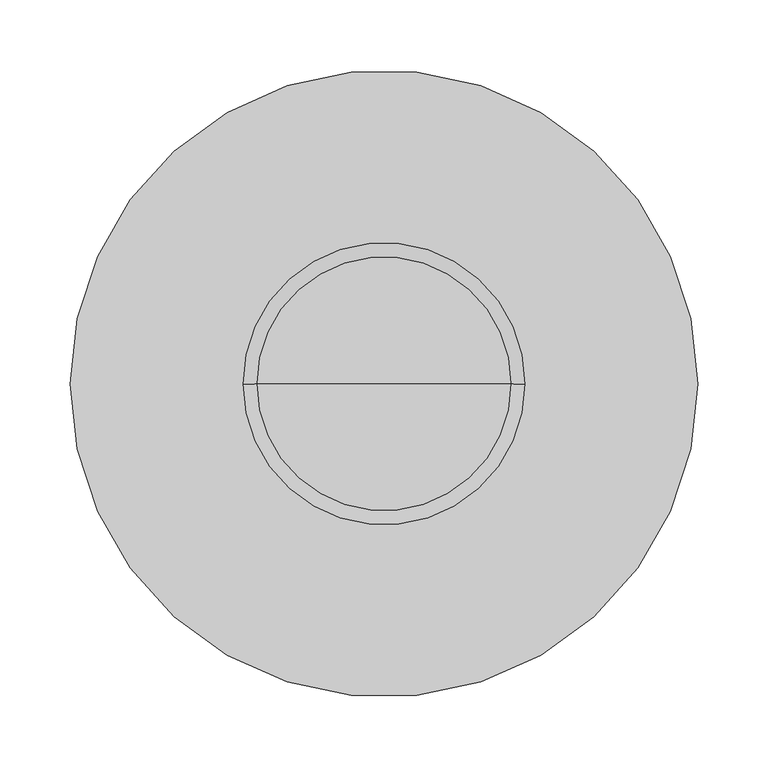
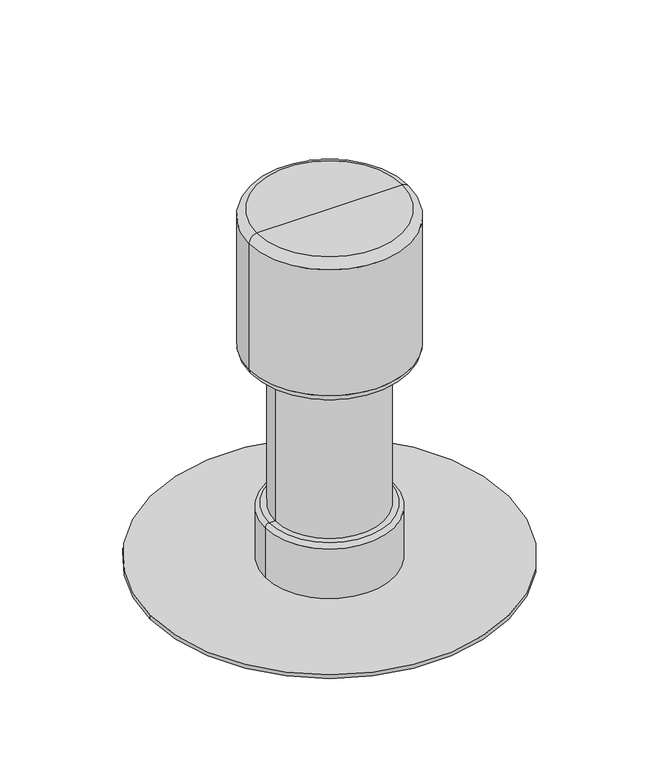
"""IFC4 building model written with IfcOpenShell, lengths in millimetres: proxy geometry, TN_Аэратор кровельный  ТехноНИКОЛЬ : Аэратор кровельный ТехноНИКОЛЬ 160х460мм."""

from ifc_helpers import new_model, si_unit, point, frame, origin, origin_with_axes, origin_2d, place, context, project, spatial, circle_curve, ellipse_curve, trimmed, segment, composite_curve, outline, extrude, source, transform, mapped, element, save
from ifc_brep_helpers import plane_surface, cylinder_surface, revolved_surface, advanced_brep


def specialty_equipment_49e8ba72(model_context):
    return source(origin(), model_context, "Body", "SolidModel", [
        advanced_brep(
        [(0.0, 0.0, 5.0), (-80.0, 0.0, 5.0), (80.0, 0.0, 5.0), (67.5, 0.0, 275.0), (-67.5, 0.0, 275.0), (0.0, 0.0, 275.0), (67.5, 0.0, 75.0), (-67.5, 0.0, 75.0), (75.0, 0.0, 75.0), (-75.0, 0.0, 75.0), (80.0, 0.0, 70.0), (-80.0, 0.0, 70.0)],
        [
            (0, 1),
            (1, 2, circle_curve(frame((0.0, 0.0, 5.0), z_axis=(0.0, 0.0, -1.0), x_axis=(-1.0, 0.0, 0.0)), 80.0)),
            (2, 0),
            (2, 1, circle_curve(frame((0.0, 0.0, 5.0), z_axis=(0.0, 0.0, -1.0), x_axis=(-1.0, 0.0, 0.0)), 80.0)),
            (3, 4, circle_curve(frame((0.0, 0.0, 275.0), z_axis=(0.0, 0.0, 1.0), x_axis=(-1.0, 0.0, 0.0)), 67.5)),
            (4, 5),
            (5, 3),
            (4, 3, circle_curve(frame((0.0, 0.0, 275.0), z_axis=(0.0, 0.0, 1.0), x_axis=(-1.0, 0.0, 0.0)), 67.5)),
            (6, 7, circle_curve(frame((0.0, 0.0, 75.0), z_axis=(0.0, 0.0, 1.0), x_axis=(-1.0, 0.0, 0.0)), 67.5)),
            (7, 4),
            (3, 6),
            (7, 6, circle_curve(frame((0.0, 0.0, 75.0), z_axis=(0.0, 0.0, 1.0), x_axis=(-1.0, 0.0, 0.0)), 67.5)),
            (8, 9, circle_curve(frame((0.0, 0.0, 75.0), z_axis=(0.0, 0.0, 1.0), x_axis=(-1.0, 0.0, 0.0)), 75.0)),
            (9, 7),
            (6, 8),
            (9, 8, circle_curve(frame((0.0, 0.0, 75.0), z_axis=(0.0, 0.0, 1.0), x_axis=(-1.0, 0.0, 0.0)), 75.0)),
            (10, 11, circle_curve(frame((0.0, 0.0, 70.0), z_axis=(0.0, 0.0, 1.0), x_axis=(-1.0, 0.0, 0.0)), 80.0)),
            (11, 9, circle_curve(frame((-75.0, 0.0, 70.0), z_axis=(0.0, 1.0, 0.0), x_axis=(1.0, 0.0, 0.0)), 5.0)),
            (8, 10, circle_curve(frame((75.0, 0.0, 70.0), z_axis=(0.0, 1.0, 0.0), x_axis=(-1.0, 0.0, 0.0)), 5.0)),
            (11, 10, circle_curve(frame((0.0, 0.0, 70.0), z_axis=(0.0, 0.0, 1.0), x_axis=(-1.0, 0.0, 0.0)), 80.0)),
            (1, 11),
            (10, 2),
        ],
        [
            plane_surface(frame((0.0, 0.0, 5.0), z_axis=(0.0, 0.0, -1.0), x_axis=(-1.0, 0.0, 0.0))),
            plane_surface(frame((0.0, 0.0, 275.0), z_axis=(0.0, 0.0, 1.0), x_axis=(-1.0, 0.0, 0.0))),
            cylinder_surface(frame((0.0, 0.0, 0.0), z_axis=(0.0, 0.0, -1.0), x_axis=(-1.0, 0.0, 0.0)), 67.5),
            plane_surface(frame((0.0, 0.0, 75.0), z_axis=(0.0, 0.0, 1.0), x_axis=(-1.0, 0.0, 0.0))),
            revolved_surface(trimmed(ellipse_curve(frame((-75.0, 0.0, 70.0), z_axis=(0.0, -1.0, 0.0), x_axis=(1.0, 0.0, 0.0)), 5.0, 5.0), [point((-75.0, 0.0, 75.0))], [point((-80.0, 0.0, 70.0))], True, "CARTESIAN"), (0.0, 0.0, 0.0), (0.0, 0.0, -1.0)),
            cylinder_surface(frame((0.0, 0.0, 0.0), z_axis=(0.0, 0.0, -1.0), x_axis=(-1.0, 0.0, 0.0)), 80.0),
        ],
        [
            (0, [[1, 2, 3]]),
            (0, [[-3, 4, -1]]),
            (1, [[5, 6, 7]]),
            (1, [[8, -7, -6]]),
            (2, [[9, 10, -5, 11]]),
            (2, [[12, -11, -8, -10]]),
            (3, [[13, 14, -9, 15]]),
            (3, [[16, -15, -12, -14]]),
            (4, [[17, 18, -13, 19]]),
            (4, [[20, -19, -16, -18]]),
            (5, [[-2, 21, -17, 22]]),
            (5, [[-4, -22, -20, -21]]),
        ],
    ),
        extrude(outline(composite_curve([segment(trimmed(circle_curve(origin_2d(), 222.5), [point((-222.5, 0.0))], [point((222.5, 0.0))], False, "CARTESIAN"), True, "CONTINUOUS"), segment(trimmed(circle_curve(origin_2d(), 222.5), [point((222.5, 0.0))], [point((-222.5, 0.0))], False, "CARTESIAN"), True, "CONTINUOUS")], self_intersect=False)), origin_with_axes(), (0.0, 0.0, 1.0), 5.0),
        advanced_brep(
        [(90.0, 0.0, 460.0), (-90.0, 0.0, 460.0), (0.0, 0.0, 460.0), (100.0, 0.0, 450.0), (-100.0, 0.0, 450.0), (100.0, 0.0, 285.0), (-100.0, 0.0, 285.0), (90.0, 0.0, 275.0), (-90.0, 0.0, 275.0), (0.0, 0.0, 275.0)],
        [
            (0, 1, circle_curve(frame((0.0, 0.0, 460.0), z_axis=(0.0, 0.0, 1.0), x_axis=(-1.0, 0.0, 0.0)), 90.0)),
            (1, 2),
            (2, 0),
            (1, 0, circle_curve(frame((0.0, 0.0, 460.0), z_axis=(0.0, 0.0, 1.0), x_axis=(-1.0, 0.0, 0.0)), 90.0)),
            (3, 4, circle_curve(frame((0.0, 0.0, 450.0), z_axis=(0.0, 0.0, 1.0), x_axis=(-1.0, 0.0, 0.0)), 100.0)),
            (4, 1, circle_curve(frame((-90.0, 0.0, 450.0), z_axis=(0.0, 1.0, 0.0), x_axis=(1.0, 0.0, 0.0)), 10.0)),
            (0, 3, circle_curve(frame((90.0, 0.0, 450.0), z_axis=(0.0, 1.0, 0.0), x_axis=(-1.0, 0.0, 0.0)), 10.0)),
            (4, 3, circle_curve(frame((0.0, 0.0, 450.0), z_axis=(0.0, 0.0, 1.0), x_axis=(-1.0, 0.0, 0.0)), 100.0)),
            (5, 6, circle_curve(frame((0.0, 0.0, 285.0), z_axis=(0.0, 0.0, 1.0), x_axis=(-1.0, 0.0, 0.0)), 100.0)),
            (6, 4),
            (3, 5),
            (6, 5, circle_curve(frame((0.0, 0.0, 285.0), z_axis=(0.0, 0.0, 1.0), x_axis=(-1.0, 0.0, 0.0)), 100.0)),
            (7, 8, circle_curve(frame((0.0, 0.0, 275.0), z_axis=(0.0, 0.0, 1.0), x_axis=(-1.0, 0.0, 0.0)), 90.0)),
            (8, 6, circle_curve(frame((-90.0, 0.0, 285.0), z_axis=(0.0, 1.0, 0.0), x_axis=(1.0, 0.0, 0.0)), 10.0)),
            (5, 7, circle_curve(frame((90.0, 0.0, 285.0), z_axis=(0.0, 1.0, 0.0), x_axis=(-1.0, 0.0, 0.0)), 10.0)),
            (8, 7, circle_curve(frame((0.0, 0.0, 275.0), z_axis=(0.0, 0.0, 1.0), x_axis=(-1.0, 0.0, 0.0)), 90.0)),
            (9, 8),
            (7, 9),
        ],
        [
            plane_surface(frame((0.0, 0.0, 460.0), z_axis=(0.0, 0.0, 1.0), x_axis=(-1.0, 0.0, 0.0))),
            revolved_surface(trimmed(ellipse_curve(frame((-90.0, 0.0, 450.0), z_axis=(0.0, -1.0, 0.0), x_axis=(1.0, 0.0, 0.0)), 10.0, 10.0), [point((-90.0, 0.0, 460.0))], [point((-100.0, 0.0, 450.0))], True, "CARTESIAN"), (0.0, 0.0, 460.0), (0.0, 0.0, -1.0)),
            cylinder_surface(frame((0.0, 0.0, 460.0), z_axis=(0.0, 0.0, -1.0), x_axis=(-1.0, 0.0, 0.0)), 100.0),
            revolved_surface(trimmed(ellipse_curve(frame((-90.0, 0.0, 285.0), z_axis=(0.0, -1.0, 0.0), x_axis=(1.0, 0.0, 0.0)), 10.0, 10.0), [point((-100.0, 0.0, 285.0))], [point((-90.0, 0.0, 275.0))], True, "CARTESIAN"), (0.0, 0.0, 460.0), (0.0, 0.0, -1.0)),
            plane_surface(frame((0.0, 0.0, 275.0), z_axis=(0.0, 0.0, -1.0), x_axis=(-1.0, 0.0, 0.0))),
        ],
        [
            (0, [[1, 2, 3]]),
            (0, [[4, -3, -2]]),
            (1, [[5, 6, -1, 7]]),
            (1, [[8, -7, -4, -6]]),
            (2, [[9, 10, -5, 11]]),
            (2, [[12, -11, -8, -10]]),
            (3, [[13, 14, -9, 15]]),
            (3, [[16, -15, -12, -14]]),
            (4, [[17, -13, 18]]),
            (4, [[-18, -16, -17]]),
        ],
    ),
    ])


if __name__ == "__main__":
    model = new_model("IFC4")
    model_context = context("Model", 3, world=origin())
    ifc_project = project(units=[si_unit("LENGTHUNIT", "METRE", prefix="MILLI")], contexts=[model_context])
    site = spatial("IfcSite", under=ifc_project)
    building = spatial("IfcBuilding", under=site)
    placement = place(None, origin())
    specialty_equipment_shape = specialty_equipment_49e8ba72(model_context)
    element("IfcBuildingElementProxy", 1, Name="TN_Аэратор кровельный  ТехноНИКОЛЬ : Аэратор кровельный ТехноНИКОЛЬ 160х460мм", ObjectType="TN_Аэратор кровельный  ТехноНИКОЛЬ : Аэратор кровельный ТехноНИКОЛЬ 160х460мм", at=placement, inside=building, context=model_context, shape_type="MappedRepresentation", body=[
        mapped(specialty_equipment_shape, transform((0.0, 0.0, 0.0), x_axis=(1.0, 0.0, 0.0), y_axis=(0.0, 1.0, 0.0), z_axis=(0.0, 0.0, 1.0))),
    ])
    save(model, "model.ifc")

# Revit data of these elements
# Type "TN_Аэратор кровельный  ТехноНИКОЛЬ : Аэратор кровельный ТехноНИКОЛЬ 160х460мм"
#   ADSK_Группирование = "Комплектующие и воронки"
#   Description = "Аэраторы кровельные ТехноНИКОЛЬ ЭКО 160х460 мм позволяют эффективно удалять излишки влаги из кровельного пирога. В системах с механическим креплением кровельного ковра к основанию рекомендуется\r\nустанавливать один аэратор на 150 м2 кровли. В кровлях устраиваемых по цементно-песчаным стяжкам с применением материалов Унифлекс ЭПВ Вент и Техноэласт ЭКВ Вент устанавливается не менее 1 аэратора на\r\n100м2. Аэраторы устанавливают равномерно по поверхности кровли. Оптимальной считается расстановка, когда большинство аэраторов установлены в местах водораздела и расстояние между аэраторами не превышает 12 м, а расстояние до паропреграждающей конструкции (парапета, деформационного шва, стены) не превышает 6м."
#   Manufacturer = "ТехноНИКОЛЬ"
#   URL = "https://shop.tn.ru/ajerator-krovel-nyj-tehnonikol-160h460-mm"
#   ADSK_Примечание = ""
#   ADSK_Обозначение = "ТехноНИКОЛЬ"
#   ADSK_Наименование = "Аэратор кровельный ТехноНИКОЛЬ 160х460мм"
#   ADSK_Марка = ""
#   ADSK_Код изделия = "34591"
#   ADSK_Завод-изготовитель = "ТехноНИКОЛЬ"
#   ADSK_Единица измерения = "шт."
#   ADSK_Группирование = "Комплектующие и воронки"
#   ADSK_URL страницы изделия = "https://shop.tn.ru/ajerator-krovel-nyj-tehnonikol-160h460-mm"
#   ADSK_URL документации изделия = "https://nav.tn.ru/upload/iblock/68a/Tekhlist-7.18_Aerator-krovelnyy-TekhnoNIKOL_rus.pdf"
#   Диаметр юбки = 445 mm
#   Высота = 460 mm
#   ADSK_Масса = 1.4
#   ADSK_Количество = 1
#   Материал = TN_ПВХ_Черный
#   Default Elevation = 0
# Element 1 (IfcBuildingElementProxy, "TN_Аэратор кровельный  ТехноНИКОЛЬ : Аэратор кровельный ТехноНИКОЛЬ 160х460мм")
#   Materials on its faces: "TN_ПВХ_Черный"
# Materials
#   "TN_ПВХ_Черный": class "Типовые", colour RGB 48 48 48, transparency 0, Cost = 0
